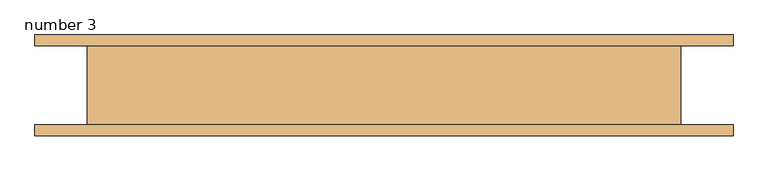
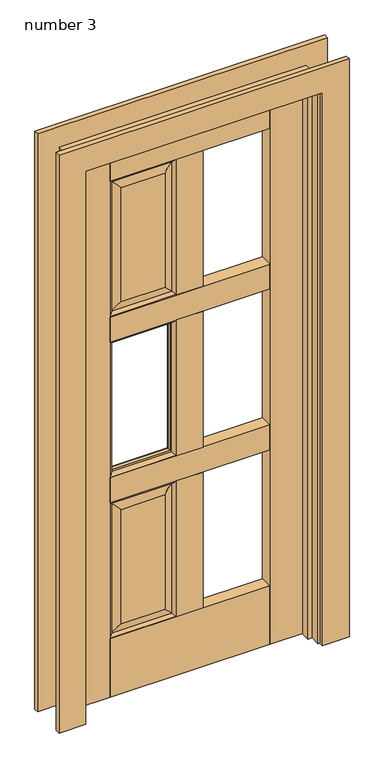
"""IFC4 building model written with IfcOpenShell, lengths in millimetres: door geometry, Door-Interior-Karona-K5660-6_Panel : number 3."""

from ifc_helpers import new_model, si_unit, frame, origin, origin_with_axes, place, context, project, spatial, polyline, ellipse_curve, outline, extrude, faceted_brep, source, transform, mapped, element, save
from ifc_brep_helpers import plane_surface, cylinder_surface, revolved_surface, advanced_brep


def number_3_e47dc6c4(model_context):
    return source(origin(), model_context, "Body", "SolidModel", [
        advanced_brep(
        [(-279.4, 15.2908, 1311.275), (-268.0746863, 24.6126, 1299.9496863), (-57.3628137, 24.6126, 1299.9496863), (-46.0375, 15.2908, 1311.275), (-57.1627, 46.3324899, 1300.1498), (-48.2727, 54.4576, 1309.0398), (-48.2727, 54.4576, 811.8602), (-57.1627, 46.3324899, 820.7502), (-268.2748, 46.3324899, 820.7502), (-277.1648, 54.4576, 811.8602), (-277.1648, 54.4576, 1309.0398), (-268.2748, 46.3324899, 1300.1498), (-46.0375, 54.4576, 809.625), (-46.0375, 15.2908, 809.625), (-279.4, 15.2908, 809.625), (-279.4, 54.4576, 809.625), (-57.1627, 34.7218, 820.7502), (-268.2748, 34.7218, 820.7502), (-47.3075, 24.6126, 1310.005), (-47.3075, 34.7218, 1310.005), (-47.3075, 34.7218, 810.895), (-47.3075, 24.6126, 810.895), (-278.13, 24.6126, 810.895), (-278.13, 24.6126, 1310.005), (-57.3628137, 24.6126, 820.9503137), (-268.0746863, 24.6126, 820.9503137), (-278.13, 34.7218, 810.895), (-279.4, 54.4576, 1311.275), (-268.2748, 34.7218, 1300.1498), (-278.13, 34.7218, 1310.005), (-46.0375, 54.4576, 1311.275), (-57.1627, 34.7218, 1300.1498)],
        [
            (0, 1, ellipse_curve(frame((-278.3689876, 25.5788135, 1310.2439876), z_axis=(0.7071067811865475, 0.0, 0.7071067811865475), x_axis=(-0.7071067811865476, 0.0, 0.7071067811865474)), 14.6223259, 10.3395458)),
            (1, 2),
            (2, 3, ellipse_curve(frame((-47.0685124, 25.5788135, 1310.2439876), z_axis=(-0.7071067811865475, 0.0, 0.7071067811865475), x_axis=(-0.7071067811865476, 0.0, -0.7071067811865474)), 14.6223259, 10.3395458)),
            (3, 0),
            (4, 5, ellipse_curve(frame((-48.2727, 45.531597, 1309.0398), z_axis=(0.7071067811865475, 0.0, -0.7071067811865475), x_axis=(0.7071067811865474, 0.0, 0.7071067811865476)), 12.6232745, 8.926003)),
            (5, 6),
            (6, 7, ellipse_curve(frame((-48.2727, 45.531597, 811.8602), z_axis=(0.7071067811865475, 0.0, 0.7071067811865475), x_axis=(-0.7071067811865474, 0.0, 0.7071067811865476)), 12.6232745, 8.926003)),
            (7, 4),
            (8, 9, ellipse_curve(frame((-277.1648, 45.531597, 811.8602), z_axis=(-0.7071067811865475, 0.0, 0.7071067811865475), x_axis=(-0.7071067811865474, 0.0, -0.7071067811865476)), 12.6232745, 8.926003)),
            (9, 10),
            (10, 11, ellipse_curve(frame((-277.1648, 45.531597, 1309.0398), z_axis=(-0.7071067811865475, 0.0, -0.7071067811865475), x_axis=(0.7071067811865474, 0.0, -0.7071067811865476)), 12.6232745, 8.926003)),
            (11, 8),
            (12, 13),
            (13, 14),
            (14, 15),
            (15, 12),
            (16, 7),
            (7, 8),
            (8, 17),
            (17, 16),
            (18, 19),
            (19, 20),
            (20, 21),
            (21, 18),
            (22, 23),
            (23, 18),
            (21, 22),
            (24, 2),
            (1, 25),
            (25, 24),
            (13, 24, ellipse_curve(frame((-47.0685124, 25.5788135, 810.6560124), z_axis=(-0.7071067811865475, 0.0, -0.7071067811865475), x_axis=(0.7071067811865476, 0.0, -0.7071067811865474)), 14.6223259, 10.3395458)),
            (25, 14, ellipse_curve(frame((-278.3689876, 25.5788135, 810.6560124), z_axis=(0.7071067811865475, 0.0, -0.7071067811865475), x_axis=(0.7071067811865476, 0.0, 0.7071067811865474)), 14.6223259, 10.3395458)),
            (20, 26),
            (26, 22),
            (14, 0),
            (0, 27),
            (27, 15),
            (11, 28),
            (28, 17),
            (26, 29),
            (29, 23),
            (3, 30),
            (30, 27),
            (11, 4),
            (4, 31),
            (31, 28),
            (29, 19),
            (3, 13),
            (12, 30),
            (16, 31),
            (5, 10),
            (9, 6),
        ],
        [
            cylinder_surface(frame((-279.4, 25.5788135, 1310.2439876), z_axis=(-1.0, 0.0, 0.0), x_axis=(0.0, -1.0, 0.0)), 10.3395458),
            cylinder_surface(frame((-48.2727, 45.531597, 1311.275), z_axis=(0.0, 0.0, 1.0), x_axis=(0.0, -1.0, 0.0)), 8.926003),
            cylinder_surface(frame((-277.1648, 45.531597, 809.625), z_axis=(0.0, 0.0, -1.0), x_axis=(0.0, -1.0, 0.0)), 8.926003),
            plane_surface(frame((-46.0375, 15.2908, 809.625), z_axis=(0.0, 0.0, -1.0), x_axis=(-1.0, 0.0, 0.0))),
            plane_surface(frame((-57.1627, 46.3324899, 820.7502), z_axis=(0.0, 0.0, 1.0), x_axis=(-1.0, 0.0, 0.0))),
            plane_surface(frame((-47.3075, 34.7218, 1310.005), z_axis=(-1.0, 0.0, 0.0), x_axis=(0.0, 0.0, -1.0))),
            plane_surface(frame((-47.3075, 24.6126, 1310.005), z_axis=(0.0, 1.0, 0.0), x_axis=(0.0, 0.0, -1.0))),
            cylinder_surface(frame((-46.0375, 25.5788135, 810.6560124), z_axis=(1.0, 0.0, 0.0), x_axis=(0.0, -1.0, 0.0)), 10.3395458),
            plane_surface(frame((-47.3075, 34.7218, 810.895), z_axis=(0.0, 0.0, 1.0), x_axis=(-1.0, 0.0, 0.0))),
            plane_surface(frame((-279.4, 15.2908, 809.625), z_axis=(-1.0, 0.0, 0.0), x_axis=(0.0, 0.0, 1.0))),
            plane_surface(frame((-268.2748, 46.3324899, 820.7502), z_axis=(1.0, 0.0, 0.0), x_axis=(0.0, 0.0, 1.0))),
            plane_surface(frame((-278.13, 34.7218, 810.895), z_axis=(1.0, 0.0, 0.0), x_axis=(0.0, 0.0, 1.0))),
            plane_surface(frame((-279.4, 15.2908, 1311.275), z_axis=(0.0, 0.0, 1.0), x_axis=(1.0, 0.0, 0.0))),
            plane_surface(frame((-268.2748, 46.3324899, 1300.1498), z_axis=(0.0, 0.0, -1.0), x_axis=(1.0, 0.0, 0.0))),
            plane_surface(frame((-278.13, 34.7218, 1310.005), z_axis=(0.0, 0.0, -1.0), x_axis=(1.0, 0.0, 0.0))),
            plane_surface(frame((-46.0375, 15.2908, 1311.275), z_axis=(1.0, 0.0, 0.0), x_axis=(0.0, 0.0, -1.0))),
            plane_surface(frame((-57.1627, 46.3324899, 1300.1498), z_axis=(-1.0, 0.0, 0.0), x_axis=(0.0, 0.0, -1.0))),
            plane_surface(frame((-57.1627, 34.7218, 1300.1498), z_axis=(0.0, -1.0, 0.0), x_axis=(0.0, 0.0, -1.0))),
            plane_surface(frame((-46.0375, 54.4576, 1311.275), z_axis=(0.0, 1.0, 0.0), x_axis=(0.0, 0.0, -1.0))),
            cylinder_surface(frame((-46.0375, 45.531597, 811.8602), z_axis=(1.0, 0.0, 0.0), x_axis=(0.0, -1.0, 0.0)), 8.926003),
            cylinder_surface(frame((-278.3689876, 25.5788135, 809.625), z_axis=(0.0, 0.0, -1.0), x_axis=(0.0, -1.0, 0.0)), 10.3395458),
            cylinder_surface(frame((-279.4, 45.531597, 1309.0398), z_axis=(-1.0, 0.0, 0.0), x_axis=(0.0, -1.0, 0.0)), 8.926003),
            cylinder_surface(frame((-47.0685124, 25.5788135, 1311.275), z_axis=(0.0, 0.0, 1.0), x_axis=(0.0, -1.0, 0.0)), 10.3395458),
        ],
        [
            (0, [[1, 2, 3, 4]]),
            (1, [[5, 6, 7, 8]]),
            (2, [[9, 10, 11, 12]]),
            (3, [[13, 14, 15, 16]]),
            (4, [[17, 18, 19, 20]]),
            (5, [[21, 22, 23, 24]]),
            (6, [[25, 26, -24, 27], [28, -2, 29, 30]]),
            (7, [[31, -30, 32, -14]]),
            (8, [[-23, 33, 34, -27]]),
            (9, [[-15, 35, 36, 37]]),
            (10, [[-19, -12, 38, 39]]),
            (11, [[-34, 40, 41, -25]]),
            (12, [[-36, -4, 42, 43]]),
            (13, [[-38, 44, 45, 46]]),
            (14, [[-41, 47, -21, -26]]),
            (15, [[-42, 48, -13, 49]]),
            (16, [[-45, -8, -17, 50]]),
            (17, [[-22, -47, -40, -33], [-39, -46, -50, -20]]),
            (18, [[-37, -43, -49, -16], [-6, 51, -10, 52]]),
            (19, [[-7, -52, -9, -18]]),
            (20, [[-32, -29, -1, -35]]),
            (21, [[-11, -51, -5, -44]]),
            (22, [[-3, -28, -31, -48]]),
        ],
    ),
        advanced_brep(
        [(-268.2748, 54.4576, 1893.8748), (-57.1627, 54.4576, 1893.8748), (-57.1627, 54.4576, 1414.4752), (-268.2748, 54.4576, 1414.4752), (-268.2748, 34.7218, 1893.8748), (-57.1627, 34.7218, 1893.8748), (-57.1627, 36.0454899, 1893.8748), (-268.2748, 36.0454899, 1893.8748), (-268.2748, 44.5515929, 1893.8748), (-57.1627, 44.5515929, 1893.8748), (-57.1627, 34.7218, 1414.4752), (-268.2748, 34.7218, 1414.4752), (-268.2748, 36.0454899, 1414.4752), (-57.1627, 36.0454899, 1414.4752), (-57.1627, 44.5515929, 1414.4752), (-268.2748, 44.5515929, 1414.4752), (-87.1686653, 44.5515929, 1863.8688347), (-238.2688347, 44.5515929, 1863.8688347), (-87.1686653, 44.5515929, 1444.4811653), (-238.2688347, 44.5515929, 1444.4811653)],
        [
            (0, 1),
            (1, 2),
            (2, 3),
            (3, 0),
            (4, 5),
            (5, 6),
            (6, 7),
            (7, 4),
            (0, 8),
            (8, 9),
            (9, 1),
            (10, 11),
            (11, 12),
            (12, 13),
            (13, 10),
            (2, 14),
            (14, 15),
            (15, 3),
            (15, 8),
            (11, 4),
            (7, 12),
            (9, 14),
            (5, 10),
            (13, 6),
            (16, 17),
            (17, 7, ellipse_curve(frame((-270.2131685, 100.0605261, 1895.8131685), z_axis=(-0.7071067811865475, 0.0, -0.7071067811865475), x_axis=(-0.7071067811865476, 0.0, 0.7071067811865474)), 90.5724254, 64.0443762)),
            (6, 16, ellipse_curve(frame((-55.2243315, 100.0605261, 1895.8131685), z_axis=(0.7071067811865475, 0.0, -0.7071067811865475), x_axis=(-0.7071067811865476, 0.0, -0.7071067811865474)), 90.5724254, 64.0443762)),
            (18, 16),
            (13, 18, ellipse_curve(frame((-55.2243315, 100.0605261, 1412.5368315), z_axis=(-0.7071067811865475, 0.0, -0.7071067811865475), x_axis=(-0.7071067811865474, 0.0, 0.7071067811865476)), 90.5724254, 64.0443762)),
            (19, 18),
            (12, 19, ellipse_curve(frame((-270.2131685, 100.0605261, 1412.5368315), z_axis=(-0.7071067811865475, 0.0, 0.7071067811865475), x_axis=(0.7071067811865476, 0.0, 0.7071067811865474)), 90.5724254, 64.0443762)),
            (17, 19),
        ],
        [
            plane_surface(frame((-57.1627, 54.4576, 1893.8748), z_axis=(0.0, 1.0, 0.0), x_axis=(0.0, 0.0, -1.0))),
            plane_surface(frame((-57.1627, 34.7218, 1893.8748), z_axis=(0.0, 0.0, 1.0), x_axis=(1.0, 0.0, 0.0))),
            plane_surface(frame((-57.1627, 34.7218, 1414.4752), z_axis=(0.0, 0.0, -1.0), x_axis=(-1.0, 0.0, 0.0))),
            plane_surface(frame((-268.2748, 54.4576, 1893.8748), z_axis=(-1.0, 0.0, 0.0), x_axis=(0.0, 0.0, -1.0))),
            plane_surface(frame((-57.1627, 34.7218, 1893.8748), z_axis=(1.0, 0.0, 0.0), x_axis=(0.0, 0.0, -1.0))),
            plane_surface(frame((-268.2748, 34.7218, 1893.8748), z_axis=(0.0, -1.0, 0.0), x_axis=(0.0, 0.0, -1.0))),
            revolved_surface(polyline([(-334.2575446888527, 100.0605261, 1831.7687923), (8.820044688852704, 100.0605261, 1831.7687923)]), (-279.4, 100.0605261, 1895.8131685), (-1.0, 0.0, 0.0)),
            revolved_surface(polyline([(-119.2687077, 100.0605261, 1959.8575446888528), (-119.2687077, 100.0605261, 1348.4924553111473)]), (-55.2243315, 100.0605261, 1905.0), (0.0, 0.0, 1.0)),
            revolved_surface(polyline([(8.820044688852683, 100.0605261, 1476.5812077), (-334.2575446888527, 100.0605261, 1476.5812077)]), (-46.0375, 100.0605261, 1412.5368315), (1.0, 0.0, 0.0)),
            revolved_surface(polyline([(-206.1687923, 100.0605261, 1348.4924553111473), (-206.1687923, 100.0605261, 1959.8575446888526)]), (-270.2131685, 100.0605261, 1403.35), (0.0, 0.0, -1.0)),
            plane_surface(frame((-279.4, 44.5515929, 1403.35), z_axis=(0.0, -1.0, 0.0), x_axis=(0.0, 0.0, 1.0))),
        ],
        [
            (0, [[1, 2, 3, 4]]),
            (1, [[5, 6, 7, 8]]),
            (1, [[-1, 9, 10, 11]]),
            (2, [[12, 13, 14, 15]]),
            (2, [[-3, 16, 17, 18]]),
            (3, [[-4, -18, 19, -9]]),
            (3, [[20, -8, 21, -13]]),
            (4, [[-2, -11, 22, -16]]),
            (4, [[23, -15, 24, -6]]),
            (5, [[-5, -20, -12, -23]]),
            (6, [[25, 26, -7, 27]]),
            (7, [[28, -27, -24, 29]]),
            (8, [[30, -29, -14, 31]]),
            (9, [[32, -31, -21, -26]]),
            (10, [[-10, -19, -17, -22], [-25, -28, -30, -32]]),
        ],
    ),
        advanced_brep(
        [(-268.2748, 24.6126, 1893.8748), (-57.1627, 24.6126, 1893.8748), (-57.1627, 24.6126, 1414.4752), (-268.2748, 24.6126, 1414.4752), (-239.4448579, 15.4432, 1443.3051421), (-85.9926421, 15.4432, 1443.3051421), (-85.9926421, 15.4432, 1865.0448579), (-239.4448579, 15.4432, 1865.0448579), (-268.2748, 23.2889101, 1893.8748), (-57.1627, 23.2889101, 1893.8748), (-57.1627, 23.2889101, 1414.4752), (-268.2748, 23.2889101, 1414.4752)],
        [
            (0, 1),
            (1, 2),
            (2, 3),
            (3, 0),
            (4, 5),
            (5, 6),
            (6, 7),
            (7, 4),
            (0, 8),
            (8, 9),
            (9, 1),
            (2, 10),
            (10, 11),
            (11, 3),
            (4, 11, ellipse_curve(frame((-270.2131685, -40.7261261, 1412.5368315), z_axis=(-0.7071067811865475, 0.0, 0.7071067811865475), x_axis=(0.7071067811865476, 0.0, 0.7071067811865474)), 90.5724254, 64.0443762)),
            (10, 5, ellipse_curve(frame((-55.2243315, -40.7261261, 1412.5368315), z_axis=(0.7071067811865475, 0.0, 0.7071067811865475), x_axis=(0.7071067811865476, 0.0, -0.7071067811865474)), 90.5724254, 64.0443762)),
            (7, 8, ellipse_curve(frame((-270.2131685, -40.7261261, 1895.8131685), z_axis=(0.7071067811865475, 0.0, 0.7071067811865475), x_axis=(0.7071067811865474, 0.0, -0.7071067811865476)), 90.5724254, 64.0443762)),
            (8, 11),
            (6, 9, ellipse_curve(frame((-55.2243315, -40.7261261, 1895.8131685), z_axis=(0.7071067811865475, 0.0, -0.7071067811865475), x_axis=(-0.7071067811865476, 0.0, -0.7071067811865474)), 90.5724254, 64.0443762)),
            (10, 9),
        ],
        [
            plane_surface(frame((-57.1627, 24.6126, 1893.8748), z_axis=(0.0, 1.0, 0.0), x_axis=(0.0, 0.0, -1.0))),
            plane_surface(frame((-268.2748, 15.4432, 1893.8748), z_axis=(0.0, -1.0, 0.0), x_axis=(0.0, 0.0, -1.0))),
            plane_surface(frame((-57.1627, 34.7218, 1893.8748), z_axis=(0.0, 0.0, 1.0), x_axis=(1.0, 0.0, 0.0))),
            plane_surface(frame((-57.1627, 34.7218, 1414.4752), z_axis=(0.0, 0.0, -1.0), x_axis=(-1.0, 0.0, 0.0))),
            revolved_surface(polyline([(8.820044688852711, -40.7261261, 1476.5812077), (-334.2575446888527, -40.7261261, 1476.5812077)]), (-46.0375, -40.7261261, 1412.5368315), (1.0, 0.0, 0.0)),
            revolved_surface(polyline([(-206.1687923, -40.7261261, 1348.4924553111473), (-206.1687923, -40.7261261, 1959.8575446888528)]), (-270.2131685, -40.7261261, 1403.35), (0.0, 0.0, -1.0)),
            revolved_surface(polyline([(-334.2575446888527, -40.7261261, 1831.7687923), (8.820044688852704, -40.7261261, 1831.7687923)]), (-279.4, -40.7261261, 1895.8131685), (-1.0, 0.0, 0.0)),
            revolved_surface(polyline([(-119.2687077, -40.7261261, 1959.8575446888528), (-119.2687077, -40.7261261, 1348.4924553111473)]), (-55.2243315, -40.7261261, 1905.0), (0.0, 0.0, 1.0)),
            plane_surface(frame((-268.2748, 24.6126, 1893.8748), z_axis=(-1.0, 0.0, 0.0), x_axis=(0.0, 0.0, -1.0))),
            plane_surface(frame((-57.1627, 15.4432, 1893.8748), z_axis=(1.0, 0.0, 0.0), x_axis=(0.0, 0.0, -1.0))),
        ],
        [
            (0, [[1, 2, 3, 4]]),
            (1, [[5, 6, 7, 8]]),
            (2, [[-1, 9, 10, 11]]),
            (3, [[-3, 12, 13, 14]]),
            (4, [[15, -13, 16, -5]]),
            (5, [[-15, -8, 17, 18]]),
            (6, [[-17, -7, 19, -10]]),
            (7, [[-19, -6, -16, 20]]),
            (8, [[-4, -14, -18, -9]]),
            (9, [[-2, -11, -20, -12]]),
        ],
    ),
        advanced_brep(
        [(-279.4, 15.2908, 1905.0), (-268.0746863, 24.6126, 1893.6746863), (-57.3628137, 24.6126, 1893.6746863), (-46.0375, 15.2908, 1905.0), (-57.1627, 46.3324899, 1893.8748), (-48.2727, 54.4576, 1902.7648), (-48.2727, 54.4576, 1405.5852), (-57.1627, 46.3324899, 1414.4752), (-268.2748, 46.3324899, 1414.4752), (-277.1648, 54.4576, 1405.5852), (-277.1648, 54.4576, 1902.7648), (-268.2748, 46.3324899, 1893.8748), (-46.0375, 54.4576, 1403.35), (-46.0375, 15.2908, 1403.35), (-279.4, 15.2908, 1403.35), (-279.4, 54.4576, 1403.35), (-57.1627, 34.7218, 1414.4752), (-268.2748, 34.7218, 1414.4752), (-47.3075, 24.6126, 1903.73), (-47.3075, 34.7218, 1903.73), (-47.3075, 34.7218, 1404.62), (-47.3075, 24.6126, 1404.62), (-278.13, 24.6126, 1404.62), (-278.13, 24.6126, 1903.73), (-57.3628137, 24.6126, 1414.6753137), (-268.0746863, 24.6126, 1414.6753137), (-278.13, 34.7218, 1404.62), (-279.4, 54.4576, 1905.0), (-268.2748, 34.7218, 1893.8748), (-278.13, 34.7218, 1903.73), (-46.0375, 54.4576, 1905.0), (-57.1627, 34.7218, 1893.8748)],
        [
            (0, 1, ellipse_curve(frame((-278.3689876, 25.5788135, 1903.9689876), z_axis=(0.7071067811865475, 0.0, 0.7071067811865475), x_axis=(-0.7071067811865476, 0.0, 0.7071067811865474)), 14.6223259, 10.3395458)),
            (1, 2),
            (2, 3, ellipse_curve(frame((-47.0685124, 25.5788135, 1903.9689876), z_axis=(-0.7071067811865475, 0.0, 0.7071067811865475), x_axis=(-0.7071067811865476, 0.0, -0.7071067811865474)), 14.6223259, 10.3395458)),
            (3, 0),
            (4, 5, ellipse_curve(frame((-48.2727, 45.531597, 1902.7648), z_axis=(0.7071067811865475, 0.0, -0.7071067811865475), x_axis=(0.7071067811865474, 0.0, 0.7071067811865476)), 12.6232745, 8.926003)),
            (5, 6),
            (6, 7, ellipse_curve(frame((-48.2727, 45.531597, 1405.5852), z_axis=(0.7071067811865475, 0.0, 0.7071067811865475), x_axis=(-0.7071067811865474, 0.0, 0.7071067811865476)), 12.6232745, 8.926003)),
            (7, 4),
            (8, 9, ellipse_curve(frame((-277.1648, 45.531597, 1405.5852), z_axis=(-0.7071067811865475, 0.0, 0.7071067811865475), x_axis=(-0.7071067811865474, 0.0, -0.7071067811865476)), 12.6232745, 8.926003)),
            (9, 10),
            (10, 11, ellipse_curve(frame((-277.1648, 45.531597, 1902.7648), z_axis=(-0.7071067811865475, 0.0, -0.7071067811865475), x_axis=(0.7071067811865474, 0.0, -0.7071067811865476)), 12.6232745, 8.926003)),
            (11, 8),
            (12, 13),
            (13, 14),
            (14, 15),
            (15, 12),
            (16, 7),
            (7, 8),
            (8, 17),
            (17, 16),
            (18, 19),
            (19, 20),
            (20, 21),
            (21, 18),
            (22, 23),
            (23, 18),
            (21, 22),
            (24, 2),
            (1, 25),
            (25, 24),
            (13, 24, ellipse_curve(frame((-47.0685124, 25.5788135, 1404.3810124), z_axis=(-0.7071067811865475, 0.0, -0.7071067811865475), x_axis=(0.7071067811865476, 0.0, -0.7071067811865474)), 14.6223259, 10.3395458)),
            (25, 14, ellipse_curve(frame((-278.3689876, 25.5788135, 1404.3810124), z_axis=(0.7071067811865475, 0.0, -0.7071067811865475), x_axis=(0.7071067811865476, 0.0, 0.7071067811865474)), 14.6223259, 10.3395458)),
            (20, 26),
            (26, 22),
            (14, 0),
            (0, 27),
            (27, 15),
            (11, 28),
            (28, 17),
            (26, 29),
            (29, 23),
            (3, 30),
            (30, 27),
            (11, 4),
            (4, 31),
            (31, 28),
            (29, 19),
            (3, 13),
            (12, 30),
            (16, 31),
            (5, 10),
            (9, 6),
        ],
        [
            cylinder_surface(frame((-279.4, 25.5788135, 1903.9689876), z_axis=(-1.0, 0.0, 0.0), x_axis=(0.0, -1.0, 0.0)), 10.3395458),
            cylinder_surface(frame((-48.2727, 45.531597, 1905.0), z_axis=(0.0, 0.0, 1.0), x_axis=(0.0, -1.0, 0.0)), 8.926003),
            cylinder_surface(frame((-277.1648, 45.531597, 1403.35), z_axis=(0.0, 0.0, -1.0), x_axis=(0.0, -1.0, 0.0)), 8.926003),
            plane_surface(frame((-46.0375, 15.2908, 1403.35), z_axis=(0.0, 0.0, -1.0), x_axis=(-1.0, 0.0, 0.0))),
            plane_surface(frame((-57.1627, 46.3324899, 1414.4752), z_axis=(0.0, 0.0, 1.0), x_axis=(-1.0, 0.0, 0.0))),
            plane_surface(frame((-47.3075, 34.7218, 1903.73), z_axis=(-1.0, 0.0, 0.0), x_axis=(0.0, 0.0, -1.0))),
            plane_surface(frame((-47.3075, 24.6126, 1903.73), z_axis=(0.0, 1.0, 0.0), x_axis=(0.0, 0.0, -1.0))),
            cylinder_surface(frame((-46.0375, 25.5788135, 1404.3810124), z_axis=(1.0, 0.0, 0.0), x_axis=(0.0, -1.0, 0.0)), 10.3395458),
            plane_surface(frame((-47.3075, 34.7218, 1404.62), z_axis=(0.0, 0.0, 1.0), x_axis=(-1.0, 0.0, 0.0))),
            plane_surface(frame((-279.4, 15.2908, 1403.35), z_axis=(-1.0, 0.0, 0.0), x_axis=(0.0, 0.0, 1.0))),
            plane_surface(frame((-268.2748, 46.3324899, 1414.4752), z_axis=(1.0, 0.0, 0.0), x_axis=(0.0, 0.0, 1.0))),
            plane_surface(frame((-278.13, 34.7218, 1404.62), z_axis=(1.0, 0.0, 0.0), x_axis=(0.0, 0.0, 1.0))),
            plane_surface(frame((-279.4, 15.2908, 1905.0), z_axis=(0.0, 0.0, 1.0), x_axis=(1.0, 0.0, 0.0))),
            plane_surface(frame((-268.2748, 46.3324899, 1893.8748), z_axis=(0.0, 0.0, -1.0), x_axis=(1.0, 0.0, 0.0))),
            plane_surface(frame((-278.13, 34.7218, 1903.73), z_axis=(0.0, 0.0, -1.0), x_axis=(1.0, 0.0, 0.0))),
            plane_surface(frame((-46.0375, 15.2908, 1905.0), z_axis=(1.0, 0.0, 0.0), x_axis=(0.0, 0.0, -1.0))),
            plane_surface(frame((-57.1627, 46.3324899, 1893.8748), z_axis=(-1.0, 0.0, 0.0), x_axis=(0.0, 0.0, -1.0))),
            plane_surface(frame((-57.1627, 34.7218, 1893.8748), z_axis=(0.0, -1.0, 0.0), x_axis=(0.0, 0.0, -1.0))),
            plane_surface(frame((-46.0375, 54.4576, 1905.0), z_axis=(0.0, 1.0, 0.0), x_axis=(0.0, 0.0, -1.0))),
            cylinder_surface(frame((-46.0375, 45.531597, 1405.5852), z_axis=(1.0, 0.0, 0.0), x_axis=(0.0, -1.0, 0.0)), 8.926003),
            cylinder_surface(frame((-278.3689876, 25.5788135, 1403.35), z_axis=(0.0, 0.0, -1.0), x_axis=(0.0, -1.0, 0.0)), 10.3395458),
            cylinder_surface(frame((-279.4, 45.531597, 1902.7648), z_axis=(-1.0, 0.0, 0.0), x_axis=(0.0, -1.0, 0.0)), 8.926003),
            cylinder_surface(frame((-47.0685124, 25.5788135, 1905.0), z_axis=(0.0, 0.0, 1.0), x_axis=(0.0, -1.0, 0.0)), 10.3395458),
        ],
        [
            (0, [[1, 2, 3, 4]]),
            (1, [[5, 6, 7, 8]]),
            (2, [[9, 10, 11, 12]]),
            (3, [[13, 14, 15, 16]]),
            (4, [[17, 18, 19, 20]]),
            (5, [[21, 22, 23, 24]]),
            (6, [[25, 26, -24, 27], [28, -2, 29, 30]]),
            (7, [[31, -30, 32, -14]]),
            (8, [[-23, 33, 34, -27]]),
            (9, [[-15, 35, 36, 37]]),
            (10, [[-19, -12, 38, 39]]),
            (11, [[-34, 40, 41, -25]]),
            (12, [[-36, -4, 42, 43]]),
            (13, [[-38, 44, 45, 46]]),
            (14, [[-41, 47, -21, -26]]),
            (15, [[-42, 48, -13, 49]]),
            (16, [[-45, -8, -17, 50]]),
            (17, [[-22, -47, -40, -33], [-39, -46, -50, -20]]),
            (18, [[-37, -43, -49, -16], [-6, 51, -10, 52]]),
            (19, [[-7, -52, -9, -18]]),
            (20, [[-32, -29, -1, -35]]),
            (21, [[-11, -51, -5, -44]]),
            (22, [[-3, -28, -31, -48]]),
        ],
    ),
        advanced_brep(
        [(-268.2748, 34.7218, 706.4248), (-57.1627, 34.7218, 706.4248), (-57.1627, 36.0454899, 706.4248), (-268.2748, 36.0454899, 706.4248), (-57.1627, 54.4576, 706.4248), (-268.2748, 54.4576, 706.4248), (-268.2748, 44.5515929, 706.4248), (-57.1627, 44.5515929, 706.4248), (-57.1627, 34.7218, 227.0252), (-268.2748, 34.7218, 227.0252), (-268.2748, 36.0454899, 227.0252), (-57.1627, 36.0454899, 227.0252), (-268.2748, 54.4576, 227.0252), (-57.1627, 54.4576, 227.0252), (-57.1627, 44.5515929, 227.0252), (-268.2748, 44.5515929, 227.0252), (-87.1686653, 44.5515929, 676.4188347), (-238.2688347, 44.5515929, 676.4188347), (-87.1686653, 44.5515929, 257.0311653), (-238.2688347, 44.5515929, 257.0311653)],
        [
            (0, 1),
            (1, 2),
            (2, 3),
            (3, 0),
            (4, 5),
            (5, 6),
            (6, 7),
            (7, 4),
            (8, 9),
            (9, 10),
            (10, 11),
            (11, 8),
            (12, 13),
            (13, 14),
            (14, 15),
            (15, 12),
            (5, 12),
            (15, 6),
            (9, 0),
            (3, 10),
            (4, 13),
            (7, 14),
            (1, 8),
            (11, 2),
            (16, 17),
            (17, 3, ellipse_curve(frame((-270.2131685, 100.0605261, 708.3631685), z_axis=(-0.7071067811865475, 0.0, -0.7071067811865475), x_axis=(-0.7071067811865476, 0.0, 0.7071067811865474)), 90.5724254, 64.0443762)),
            (2, 16, ellipse_curve(frame((-55.2243315, 100.0605261, 708.3631685), z_axis=(0.7071067811865475, 0.0, -0.7071067811865475), x_axis=(-0.7071067811865476, 0.0, -0.7071067811865474)), 90.5724254, 64.0443762)),
            (18, 16),
            (11, 18, ellipse_curve(frame((-55.2243315, 100.0605261, 225.0868315), z_axis=(-0.7071067811865475, 0.0, -0.7071067811865475), x_axis=(-0.7071067811865474, 0.0, 0.7071067811865476)), 90.5724254, 64.0443762)),
            (19, 18),
            (10, 19, ellipse_curve(frame((-270.2131685, 100.0605261, 225.0868315), z_axis=(-0.7071067811865475, 0.0, 0.7071067811865475), x_axis=(0.7071067811865476, 0.0, 0.7071067811865474)), 90.5724254, 64.0443762)),
            (17, 19),
        ],
        [
            plane_surface(frame((-57.1627, 34.7218, 706.4248), z_axis=(0.0, 0.0, 1.0), x_axis=(1.0, 0.0, 0.0))),
            plane_surface(frame((-57.1627, 34.7218, 227.0252), z_axis=(0.0, 0.0, -1.0), x_axis=(-1.0, 0.0, 0.0))),
            plane_surface(frame((-268.2748, 54.4576, 706.4248), z_axis=(-1.0, 0.0, 0.0), x_axis=(0.0, 0.0, -1.0))),
            plane_surface(frame((-57.1627, 54.4576, 706.4248), z_axis=(0.0, 1.0, 0.0), x_axis=(0.0, 0.0, -1.0))),
            plane_surface(frame((-57.1627, 34.7218, 706.4248), z_axis=(1.0, 0.0, 0.0), x_axis=(0.0, 0.0, -1.0))),
            plane_surface(frame((-268.2748, 34.7218, 706.4248), z_axis=(0.0, -1.0, 0.0), x_axis=(0.0, 0.0, -1.0))),
            revolved_surface(polyline([(-334.2575446888527, 100.0605261, 644.3187923), (8.820044688852704, 100.0605261, 644.3187923)]), (-279.4, 100.0605261, 708.3631685), (-1.0, 0.0, 0.0)),
            revolved_surface(polyline([(-119.2687077, 100.0605261, 772.4075446888527), (-119.2687077, 100.0605261, 161.04245531114725)]), (-55.2243315, 100.0605261, 717.55), (0.0, 0.0, 1.0)),
            revolved_surface(polyline([(8.820044688852683, 100.0605261, 289.1312077), (-334.2575446888527, 100.0605261, 289.1312077)]), (-46.0375, 100.0605261, 225.0868315), (1.0, 0.0, 0.0)),
            revolved_surface(polyline([(-206.1687923, 100.0605261, 161.0424553111473), (-206.1687923, 100.0605261, 772.4075446888527)]), (-270.2131685, 100.0605261, 215.9), (0.0, 0.0, -1.0)),
            plane_surface(frame((-279.4, 44.5515929, 215.9), z_axis=(0.0, -1.0, 0.0), x_axis=(0.0, 0.0, 1.0))),
        ],
        [
            (0, [[1, 2, 3, 4]]),
            (0, [[5, 6, 7, 8]]),
            (1, [[9, 10, 11, 12]]),
            (1, [[13, 14, 15, 16]]),
            (2, [[17, -16, 18, -6]]),
            (2, [[19, -4, 20, -10]]),
            (3, [[-5, 21, -13, -17]]),
            (4, [[-21, -8, 22, -14]]),
            (4, [[23, -12, 24, -2]]),
            (5, [[-1, -19, -9, -23]]),
            (6, [[25, 26, -3, 27]]),
            (7, [[28, -27, -24, 29]]),
            (8, [[30, -29, -11, 31]]),
            (9, [[32, -31, -20, -26]]),
            (10, [[-7, -18, -15, -22], [-25, -28, -30, -32]]),
        ],
    ),
        advanced_brep(
        [(-57.1627, 24.6126, 706.4248), (-268.2748, 24.6126, 706.4248), (-268.2748, 23.2889101, 706.4248), (-57.1627, 23.2889101, 706.4248), (-268.2748, 24.6126, 227.0252), (-57.1627, 24.6126, 227.0252), (-57.1627, 23.2889101, 227.0252), (-268.2748, 23.2889101, 227.0252), (-239.4448579, 15.4432, 255.8551421), (-85.9926421, 15.4432, 255.8551421), (-85.9926421, 15.4432, 677.5948579), (-239.4448579, 15.4432, 677.5948579)],
        [
            (0, 1),
            (1, 2),
            (2, 3),
            (3, 0),
            (4, 5),
            (5, 6),
            (6, 7),
            (7, 4),
            (0, 5),
            (4, 1),
            (8, 9),
            (9, 10),
            (10, 11),
            (11, 8),
            (8, 7, ellipse_curve(frame((-270.2131685, -40.7261261, 225.0868315), z_axis=(-0.7071067811865475, 0.0, 0.7071067811865475), x_axis=(0.7071067811865476, 0.0, 0.7071067811865474)), 90.5724254, 64.0443762)),
            (6, 9, ellipse_curve(frame((-55.2243315, -40.7261261, 225.0868315), z_axis=(0.7071067811865475, 0.0, 0.7071067811865475), x_axis=(0.7071067811865476, 0.0, -0.7071067811865474)), 90.5724254, 64.0443762)),
            (11, 2, ellipse_curve(frame((-270.2131685, -40.7261261, 708.3631685), z_axis=(0.7071067811865475, 0.0, 0.7071067811865475), x_axis=(0.7071067811865474, 0.0, -0.7071067811865476)), 90.5724254, 64.0443762)),
            (2, 7),
            (10, 3, ellipse_curve(frame((-55.2243315, -40.7261261, 708.3631685), z_axis=(0.7071067811865475, 0.0, -0.7071067811865475), x_axis=(-0.7071067811865476, 0.0, -0.7071067811865474)), 90.5724254, 64.0443762)),
            (6, 3),
        ],
        [
            plane_surface(frame((-57.1627, 34.7218, 706.4248), z_axis=(0.0, 0.0, 1.0), x_axis=(1.0, 0.0, 0.0))),
            plane_surface(frame((-57.1627, 34.7218, 227.0252), z_axis=(0.0, 0.0, -1.0), x_axis=(-1.0, 0.0, 0.0))),
            plane_surface(frame((-57.1627, 24.6126, 706.4248), z_axis=(0.0, 1.0, 0.0), x_axis=(0.0, 0.0, -1.0))),
            plane_surface(frame((-268.2748, 15.4432, 706.4248), z_axis=(0.0, -1.0, 0.0), x_axis=(0.0, 0.0, -1.0))),
            revolved_surface(polyline([(8.820044688852711, -40.7261261, 289.1312077), (-334.2575446888527, -40.7261261, 289.1312077)]), (-46.0375, -40.7261261, 225.0868315), (1.0, 0.0, 0.0)),
            revolved_surface(polyline([(-206.1687923, -40.7261261, 161.0424553111473), (-206.1687923, -40.7261261, 772.4075446888527)]), (-270.2131685, -40.7261261, 215.9), (0.0, 0.0, -1.0)),
            revolved_surface(polyline([(-334.2575446888527, -40.7261261, 644.3187923), (8.820044688852704, -40.7261261, 644.3187923)]), (-279.4, -40.7261261, 708.3631685), (-1.0, 0.0, 0.0)),
            revolved_surface(polyline([(-119.2687077, -40.7261261, 772.4075446888527), (-119.2687077, -40.7261261, 161.04245531114736)]), (-55.2243315, -40.7261261, 717.55), (0.0, 0.0, 1.0)),
            plane_surface(frame((-268.2748, 24.6126, 706.4248), z_axis=(-1.0, 0.0, 0.0), x_axis=(0.0, 0.0, -1.0))),
            plane_surface(frame((-57.1627, 15.4432, 706.4248), z_axis=(1.0, 0.0, 0.0), x_axis=(0.0, 0.0, -1.0))),
        ],
        [
            (0, [[1, 2, 3, 4]]),
            (1, [[5, 6, 7, 8]]),
            (2, [[-1, 9, -5, 10]]),
            (3, [[11, 12, 13, 14]]),
            (4, [[15, -7, 16, -11]]),
            (5, [[-15, -14, 17, 18]]),
            (6, [[-17, -13, 19, -3]]),
            (7, [[-19, -12, -16, 20]]),
            (8, [[-10, -8, -18, -2]]),
            (9, [[-9, -4, -20, -6]]),
        ],
    ),
        advanced_brep(
        [(-279.4, 15.2908, 717.55), (-268.0746863, 24.6126, 706.2246863), (-57.3628137, 24.6126, 706.2246863), (-46.0375, 15.2908, 717.55), (-57.1627, 46.3324899, 706.4248), (-48.2727, 54.4576, 715.3148), (-48.2727, 54.4576, 218.1352), (-57.1627, 46.3324899, 227.0252), (-279.4, 54.4576, 215.9), (-279.4, 54.4576, 717.55), (-46.0375, 54.4576, 717.55), (-46.0375, 54.4576, 215.9), (-277.1648, 54.4576, 715.3148), (-277.1648, 54.4576, 218.1352), (-46.0375, 15.2908, 215.9), (-279.4, 15.2908, 215.9), (-57.1627, 34.7218, 227.0252), (-268.2748, 46.3324899, 227.0252), (-268.2748, 34.7218, 227.0252), (-47.3075, 24.6126, 217.17), (-47.3075, 34.7218, 217.17), (-278.13, 34.7218, 217.17), (-278.13, 24.6126, 217.17), (-268.2748, 46.3324899, 706.4248), (-268.2748, 34.7218, 706.4248), (-278.13, 34.7218, 716.28), (-278.13, 24.6126, 716.28), (-57.1627, 34.7218, 706.4248), (-47.3075, 34.7218, 716.28), (-47.3075, 24.6126, 716.28), (-57.3628137, 24.6126, 227.2253137), (-268.0746863, 24.6126, 227.2253137)],
        [
            (0, 1, ellipse_curve(frame((-278.3689876, 25.5788135, 716.5189876), z_axis=(0.7071067811865475, 0.0, 0.7071067811865475), x_axis=(-0.7071067811865476, 0.0, 0.7071067811865474)), 14.6223259, 10.3395458)),
            (1, 2),
            (2, 3, ellipse_curve(frame((-47.0685124, 25.5788135, 716.5189876), z_axis=(-0.7071067811865475, 0.0, 0.7071067811865475), x_axis=(-0.7071067811865476, 0.0, -0.7071067811865474)), 14.6223259, 10.3395458)),
            (3, 0),
            (4, 5, ellipse_curve(frame((-48.2727, 45.531597, 715.3148), z_axis=(0.7071067811865475, 0.0, -0.7071067811865475), x_axis=(0.7071067811865474, 0.0, 0.7071067811865476)), 12.6232745, 8.926003)),
            (5, 6),
            (6, 7, ellipse_curve(frame((-48.2727, 45.531597, 218.1352), z_axis=(0.7071067811865475, 0.0, 0.7071067811865475), x_axis=(-0.7071067811865474, 0.0, 0.7071067811865476)), 12.6232745, 8.926003)),
            (7, 4),
            (8, 9),
            (9, 10),
            (10, 11),
            (11, 8),
            (5, 12),
            (12, 13),
            (13, 6),
            (11, 14),
            (14, 15),
            (15, 8),
            (16, 7),
            (7, 17),
            (17, 18),
            (18, 16),
            (19, 20),
            (20, 21),
            (21, 22),
            (22, 19),
            (15, 0),
            (0, 9),
            (17, 23),
            (23, 24),
            (24, 18),
            (21, 25),
            (25, 26),
            (26, 22),
            (3, 10),
            (23, 4),
            (4, 27),
            (27, 24),
            (25, 28),
            (28, 29),
            (29, 26),
            (3, 14),
            (16, 27),
            (20, 28),
            (19, 29),
            (30, 2),
            (1, 31),
            (31, 30),
            (30, 14, ellipse_curve(frame((-47.0685124, 25.5788135, 216.9310124), z_axis=(0.7071067811865475, 0.0, 0.7071067811865475), x_axis=(-0.7071067811865474, 0.0, 0.7071067811865476)), 14.6223259, 10.3395458)),
            (17, 13, ellipse_curve(frame((-277.1648, 45.531597, 218.1352), z_axis=(-0.7071067811865475, 0.0, 0.7071067811865475), x_axis=(-0.7071067811865474, 0.0, -0.7071067811865476)), 12.6232745, 8.926003)),
            (12, 23, ellipse_curve(frame((-277.1648, 45.531597, 715.3148), z_axis=(-0.7071067811865475, 0.0, -0.7071067811865475), x_axis=(0.7071067811865474, 0.0, -0.7071067811865476)), 12.6232745, 8.926003)),
            (31, 15, ellipse_curve(frame((-278.3689876, 25.5788135, 216.9310124), z_axis=(0.7071067811865475, 0.0, -0.7071067811865475), x_axis=(0.7071067811865476, 0.0, 0.7071067811865474)), 14.6223259, 10.3395458)),
        ],
        [
            cylinder_surface(frame((-279.4, 25.5788135, 716.5189876), z_axis=(-1.0, 0.0, 0.0), x_axis=(0.0, -1.0, 0.0)), 10.3395458),
            cylinder_surface(frame((-48.2727, 45.531597, 717.55), z_axis=(0.0, 0.0, 1.0), x_axis=(0.0, -1.0, 0.0)), 8.926003),
            plane_surface(frame((-46.0375, 54.4576, 717.55), z_axis=(0.0, 1.0, 0.0), x_axis=(0.0, 0.0, -1.0))),
            plane_surface(frame((-46.0375, 15.2908, 215.9), z_axis=(0.0, 0.0, -1.0), x_axis=(-1.0, 0.0, 0.0))),
            plane_surface(frame((-57.1627, 46.3324899, 227.0252), z_axis=(0.0, 0.0, 1.0), x_axis=(-1.0, 0.0, 0.0))),
            plane_surface(frame((-47.3075, 34.7218, 217.17), z_axis=(0.0, 0.0, 1.0), x_axis=(-1.0, 0.0, 0.0))),
            plane_surface(frame((-279.4, 15.2908, 215.9), z_axis=(-1.0, 0.0, 0.0), x_axis=(0.0, 0.0, 1.0))),
            plane_surface(frame((-268.2748, 46.3324899, 227.0252), z_axis=(1.0, 0.0, 0.0), x_axis=(0.0, 0.0, 1.0))),
            plane_surface(frame((-278.13, 34.7218, 217.17), z_axis=(1.0, 0.0, 0.0), x_axis=(0.0, 0.0, 1.0))),
            plane_surface(frame((-279.4, 15.2908, 717.55), z_axis=(0.0, 0.0, 1.0), x_axis=(1.0, 0.0, 0.0))),
            plane_surface(frame((-268.2748, 46.3324899, 706.4248), z_axis=(0.0, 0.0, -1.0), x_axis=(1.0, 0.0, 0.0))),
            plane_surface(frame((-278.13, 34.7218, 716.28), z_axis=(0.0, 0.0, -1.0), x_axis=(1.0, 0.0, 0.0))),
            plane_surface(frame((-46.0375, 15.2908, 717.55), z_axis=(1.0, 0.0, 0.0), x_axis=(0.0, 0.0, -1.0))),
            plane_surface(frame((-57.1627, 46.3324899, 706.4248), z_axis=(-1.0, 0.0, 0.0), x_axis=(0.0, 0.0, -1.0))),
            plane_surface(frame((-57.1627, 34.7218, 706.4248), z_axis=(0.0, -1.0, 0.0), x_axis=(0.0, 0.0, -1.0))),
            plane_surface(frame((-47.3075, 34.7218, 716.28), z_axis=(-1.0, 0.0, 0.0), x_axis=(0.0, 0.0, -1.0))),
            plane_surface(frame((-47.3075, 24.6126, 716.28), z_axis=(0.0, 1.0, 0.0), x_axis=(0.0, 0.0, -1.0))),
            cylinder_surface(frame((-47.0685124, 25.5788135, 717.55), z_axis=(0.0, 0.0, 1.0), x_axis=(0.0, -1.0, 0.0)), 10.3395458),
            cylinder_surface(frame((-277.1648, 45.531597, 215.9), z_axis=(0.0, 0.0, -1.0), x_axis=(0.0, -1.0, 0.0)), 8.926003),
            cylinder_surface(frame((-46.0375, 25.5788135, 216.9310124), z_axis=(1.0, 0.0, 0.0), x_axis=(0.0, -1.0, 0.0)), 10.3395458),
            cylinder_surface(frame((-46.0375, 45.531597, 218.1352), z_axis=(1.0, 0.0, 0.0), x_axis=(0.0, -1.0, 0.0)), 8.926003),
            cylinder_surface(frame((-278.3689876, 25.5788135, 215.9), z_axis=(0.0, 0.0, -1.0), x_axis=(0.0, -1.0, 0.0)), 10.3395458),
            cylinder_surface(frame((-279.4, 45.531597, 715.3148), z_axis=(-1.0, 0.0, 0.0), x_axis=(0.0, -1.0, 0.0)), 8.926003),
        ],
        [
            (0, [[1, 2, 3, 4]]),
            (1, [[5, 6, 7, 8]]),
            (2, [[9, 10, 11, 12], [-6, 13, 14, 15]]),
            (3, [[16, 17, 18, -12]]),
            (4, [[19, 20, 21, 22]]),
            (5, [[23, 24, 25, 26]]),
            (6, [[-18, 27, 28, -9]]),
            (7, [[-21, 29, 30, 31]]),
            (8, [[-25, 32, 33, 34]]),
            (9, [[-28, -4, 35, -10]]),
            (10, [[-30, 36, 37, 38]]),
            (11, [[-33, 39, 40, 41]]),
            (12, [[-35, 42, -16, -11]]),
            (13, [[-37, -8, -19, 43]]),
            (14, [[44, -39, -32, -24], [-31, -38, -43, -22]]),
            (15, [[-40, -44, -23, 45]]),
            (16, [[-34, -41, -45, -26], [46, -2, 47, 48]]),
            (17, [[-3, -46, 49, -42]]),
            (18, [[50, -14, 51, -29]]),
            (19, [[-49, -48, 52, -17]]),
            (20, [[-7, -15, -50, -20]]),
            (21, [[-52, -47, -1, -27]]),
            (22, [[-51, -13, -5, -36]]),
        ],
    ),
        extrude(outline(polyline([(279.4, 12.7), (-279.4, 12.7), (-279.4, 57.15), (279.4, 57.15), (279.4, 12.7)])), frame((0.0, 0.0, 1905.0), z_axis=(0.0, 0.0, 1.0), x_axis=(1.0, 0.0, 0.0)), (0.0, 0.0, 1.0), 127.0),
        extrude(outline(polyline([(279.4, 12.7), (-279.4, 12.7), (-279.4, 57.15), (279.4, 57.15), (279.4, 12.7)])), origin_with_axes(), (0.0, 0.0, 1.0), 215.9),
        extrude(outline(polyline([(46.0375, 12.7), (-46.0375, 12.7), (-46.0375, 57.15), (46.0375, 57.15), (46.0375, 12.7)])), frame((0.0, 0.0, 215.9), z_axis=(0.0, 0.0, 1.0), x_axis=(1.0, 0.0, 0.0)), (0.0, 0.0, 1.0), 501.65),
        extrude(outline(polyline([(46.0375, 12.7), (-46.0375, 12.7), (-46.0375, 57.15), (46.0375, 57.15), (46.0375, 12.7)])), frame((0.0, 0.0, 809.625), z_axis=(0.0, 0.0, 1.0), x_axis=(1.0, 0.0, 0.0)), (0.0, 0.0, 1.0), 501.65),
        extrude(outline(polyline([(46.0375, 12.7), (-46.0375, 12.7), (-46.0375, 57.15), (46.0375, 57.15), (46.0375, 12.7)])), frame((0.0, 0.0, 1403.35), z_axis=(0.0, 0.0, 1.0), x_axis=(1.0, 0.0, 0.0)), (0.0, 0.0, 1.0), 501.65),
        extrude(outline(polyline([(279.4, 12.7), (-279.4, 12.7), (-279.4, 57.15), (279.4, 57.15), (279.4, 12.7)])), frame((0.0, 0.0, 717.55), z_axis=(0.0, 0.0, 1.0), x_axis=(1.0, 0.0, 0.0)), (0.0, 0.0, 1.0), 92.075),
        extrude(outline(polyline([(279.4, 12.7), (-279.4, 12.7), (-279.4, 57.15), (279.4, 57.15), (279.4, 12.7)])), frame((0.0, 0.0, 1311.275), z_axis=(0.0, 0.0, 1.0), x_axis=(1.0, 0.0, 0.0)), (0.0, 0.0, 1.0), 92.075),
        extrude(outline(polyline([(406.4, 12.7), (279.4, 12.7), (279.4, 57.15), (406.4, 57.15), (406.4, 12.7)])), origin_with_axes(), (0.0, 0.0, 1.0), 2032.0),
        extrude(outline(polyline([(-279.4, 12.7), (-406.4, 12.7), (-406.4, 57.15), (-279.4, 57.15), (-279.4, 12.7)])), origin_with_axes(), (0.0, 0.0, 1.0), 2032.0),
        faceted_brep([(430.609375, -57.15, 0.0), (407.590625, -57.15, 0.0), (407.590625, -22.225, 0.0), (392.8401275, -22.225, 0.0), (392.8401275, 12.7, 0.0), (407.590625, 12.7, 0.0), (407.590625, 57.15, 0.0), (430.609375, 57.15, 0.0), (430.609375, -57.15, 2056.209375), (-430.609375, -57.15, 2056.209375), (-430.609375, -57.15, 0.0), (-407.590625, -57.15, 0.0), (-407.590625, -57.15, 2033.190625), (407.590625, -57.15, 2033.190625), (407.590625, -22.225, 2033.190625), (-407.590625, -22.225, 2033.190625), (-407.590625, -22.225, 0.0), (-392.8401275, -22.225, 0.0), (-392.8401275, -22.225, 2018.4401275), (392.8401275, -22.225, 2018.4401275), (392.8401275, 12.7, 2018.4401275), (-392.8401275, 12.7, 2018.4401275), (-392.8401275, 12.7, 0.0), (-407.590625, 12.7, 0.0), (-407.590625, 12.7, 2033.190625), (407.590625, 12.7, 2033.190625), (407.590625, 57.15, 2033.190625), (-407.590625, 57.15, 2033.190625), (-407.590625, 57.15, 0.0), (-430.609375, 57.15, 0.0), (-430.609375, 57.15, 2056.209375), (430.609375, 57.15, 2056.209375)], [[[0, 1, 2, 3, 4, 5, 6, 7]], [[1, 0, 8, 9, 10, 11, 12, 13]], [[2, 1, 13, 14]], [[3, 2, 14, 15, 16, 17, 18, 19]], [[4, 3, 19, 20]], [[5, 4, 20, 21, 22, 23, 24, 25]], [[6, 5, 25, 26]], [[7, 6, 26, 27, 28, 29, 30, 31]], [[0, 7, 31, 8]], [[14, 13, 12, 15]], [[20, 19, 18, 21]], [[26, 25, 24, 27]], [[8, 31, 30, 9]], [[10, 29, 28, 23, 22, 17, 16, 11]], [[15, 12, 11, 16]], [[21, 18, 17, 22]], [[27, 24, 23, 28]], [[9, 30, 29, 10]]]),
        extrude(outline(polyline([(2132.409375, -506.809375), (0.0, -506.809375), (0.0, -413.940625), (2039.540625, -413.940625), (2039.540625, 413.940625), (0.0, 413.940625), (0.0, 506.809375), (2132.409375, 506.809375), (2132.409375, -506.809375)])), frame((0.0, -73.025, 0.0), z_axis=(0.0, 1.0, 0.0), x_axis=(0.0, 0.0, 1.0)), (0.0, 0.0, 1.0), 15.875),
        extrude(outline(polyline([(2132.409375, 506.809375), (2132.409375, -506.809375), (0.0, -506.809375), (0.0, -413.940625), (2039.540625, -413.940625), (2039.540625, 413.940625), (0.0, 413.940625), (0.0, 506.809375), (2132.409375, 506.809375)])), frame((0.0, 57.15, 0.0), z_axis=(0.0, 1.0, 0.0), x_axis=(0.0, 0.0, 1.0)), (0.0, 0.0, 1.0), 15.875),
    ])


if __name__ == "__main__":
    model = new_model("IFC4")
    model_context = context("Model", 3, world=origin())
    ifc_project = project(units=[si_unit("LENGTHUNIT", "METRE", prefix="MILLI")], contexts=[model_context])
    site = spatial("IfcSite", under=ifc_project)
    building = spatial("IfcBuilding", under=site)
    placement = place(None, origin())
    number_3_shape = number_3_e47dc6c4(model_context)
    element("IfcDoor", 1, ObjectType="Door-Interior-Karona-K5660-6_Panel : number 3", at=placement, inside=building, context=model_context, shape_type="MappedRepresentation", body=[
        mapped(number_3_shape, transform((0.0, 0.0, 0.0), x_axis=(1.0, 0.0, 0.0), y_axis=(0.0, 1.0, 0.0), z_axis=(0.0, 0.0, 1.0))),
    ])
    save(model, "model.ifc")

# Revit data of these elements
# Type "Door-Interior-Karona-K5660-6_Panel : number 3"
#   Type Mark = "83"
#   Youtube clip = ""
#   Warranty URL = "http://www.karonadoor.com/pdf/literature/Warranty_.pdf"
#   Warranty = "Limited lifetime warranty on all interior doors."
#   Uniformat II Description = ""
#   Uniformat II Code = ""
#   Uniclass 2015 Name = "Doorsets"
#   Uniclass 2015 Code = "Pr_30_59_24"
#   Uniclass 2.0 Description = "Doorsets"
#   Uniclass 2.0 Code = "PR-59-23"
#   Uniclass 1.4 Description = "Doors"
#   Uniclass 1.4 Code = "JL20"
#   URL = "http://www.karonadoor.com/"
#   UNSPSC Code = "30171511"
#   Technical description = "http://www.karonadoor.com/pdf/Architectural.Guide.pdf"
#   Support Email = "mailto:bimsupport@jeldwen.com"
#   Region South America = "None"
#   Region Oceania = "None"
#   Region North America = "CA, US"
#   Region Middle East = "None"
#   Region Europe = "None"
#   Region Asia = "None"
#   Region Antarctica = "None"
#   Region Africa = "None"
#   QR code = "http://bimobject.com/karona/product/K5660"
#   Product url = "http://www.karonadoor.com/commercial_products.php?category_id=1&style_id=1&image_id=21"
#   Product group = "Panel Doors"
#   Product family = "Commercial Products"
#   Product data url = "https://bimobject.com/karona/product/K5660"
#   Product certification = ""
#   Product SKU = "K5660"
#   Product Guid = "0ef6a8f4-4242-4391-b579-45df545b9ddd"
#   Operation = "Swing"
#   OmniClass Description = "Wood Doors"
#   OmniClass Code = "23-17 11 15"
#   NBS Reference Description = "Doorsets"
#   NBS Reference Code = "59-23"
#   Model = "K5660"
#   Material secondary = ""
#   Material main = "Wood"
#   Masterformat 2014 Description = "Stile and Rail Wood Doors"
#   Masterformat 2014 Code = "08 14 33"
#   Manufacturer name = "Karona"
#   Manufacturer country = "United States"
#   Manufacturer = "Karona Door, Inc."
#   Keynote = "08 14 33"
#   Installation instructions = ""
#   IFC Classification = "Door"
#   Green Product Information = "Available in Certified Wood, No-added Urea, & Recycled"
#   Fire Rating Data = "http://www.karonadoor.com/pdf/literature/Fire_Door_Options.pdf"
#   Fire Rating = "Available in 20, 45, 60, & 90 minute ratings."
#   EAN code = ""
#   Design country = "United States"
#   Description = "Commercial 6-Panel Stile and Rail Wood Door"
#   Date of publishing = ""
#   COBIe Type Category = ""
#   Brand url = "http://www.karonadoor.com/"
#   BIMobject main category code = "doors"
#   BIMobject main category = "Doors"
#   BIMobject category code = "doors-swing"
#   BIMobject category = "Swing"
#   Analytic Construction = "Solid core wood"
#   Sticking Profile Note = "Select only one sticking profile."
#   Sizing Statement = "Custom sizes are available."
#   Panel Style Note = "Select only one panel style."
#   Glass Options Note = "19 styles of glass are available."
#   Fire Door Note = "Available in 20, 45, 60, & 90 minute ratings."
#   Trim Width = 0' - 3 21/32"
#   Trim Reveal = 0' - 0 1/4"
#   Trim Offset = 0' - 3"
#   Top Rail Height = 0' - 5"
#   Thermal Resistance (R) = 0.382863 (m²·K)/W
#   Stile Width = 0' - 5"
#   Sticking Offset = 0' - 0 7/16"
#   Raised Panel Offset = 0' - 1 5/8"
#   Panel Height = 1' - 7 3/4"
#   Mullion Width = 0' - 3 5/8"
#   Mid Rail Height = 4' - 7 1/4"
#   Lock Rail Width = 0' - 3 5/8"
#   Lock Rail Height = 2' - 7 7/8"
#   Jamb to Door Gap = 0' - 0 3/64"
#   Hinge Length = 0' - 2 1/4"
#   Heat Transfer Coefficient (U) = 2.6120 W/(m²·K)
#   Daylight Opening Width = 0' - 0"
#   Daylight Opening Height = 0' - 0"
#   Bottom Rail Height = 0' - 8 1/2"
#   3D Open Angle = 0.00°
#   Thickness = 0' - 1 3/4"
#   Stop Thickness = 0' - 0 1/2"
#   Stop Depth = 0' - 1 3/8"
#   Rough Width = 2' - 9 29/32"
#   Rough Height = 6' - 8 61/64"
#   Rabbet Width = 0' - 1 3/4"
#   Jamb Offset = 0' - 0 61/64"
#   Hinge Offset = 0' - 0 3/4"
#   Jamb Thickness = 0' - 0 29/32"
#   Ext. Frame Thickness = 0' - 0 5/8"
#   Int. Frame Thickness = 0' - 0 5/8"
#   Height = 6' - 8"
#   Width = 2' - 8"
#   3D Angle = 0.00°
#   Trim Visible = yes
#   Square Sticking Profile = no
#   Raised Panel Door = yes
#   Ovolo Sticking Profile = yes
#   Ogee Sticking Profile = no
#   Mission Sticking Profile = no
#   Hinge Visible = yes
#   Glass Panel Door = no
#   Flat Panel Door = no
#   Edition number = 1
#   Define Thermal Properties by = 1
#   Trim Material = Wood - Karona - Red Oak
#   Top Rail Material = Wood - Karona - Red Oak
#   Stile Material = Wood - Karona - Red Oak
#   Sticking Material = Wood - Karona - Red Oak
#   Jamb Material = Wood - Karona - Red Oak
#   Interior Panel = Wood - Karona - Red Oak
#   Door Panel Material = Wood - Karona - Red Oak
#   Bottom Rail Material = Wood - Karona - Red Oak
#   Visual Light Transmittance = 0
#   Solar Heat Gain Coefficient = 0
#   Construction Type = (empty or 0)
#   Function = (empty or 0)
#   Wall Closure = (empty or 0)
# Element 1 (IfcDoor, "Door-Interior-Karona-K5660-6_Panel : number 3")
#   Materials on its faces: "Wood - Karona - Red Oak"
# Materials
#   "Wood - Karona - Red Oak": class "Wood", colour RGB 153 121 89, transparency 0, Description = "Quercus Rubra", Cost = 0
